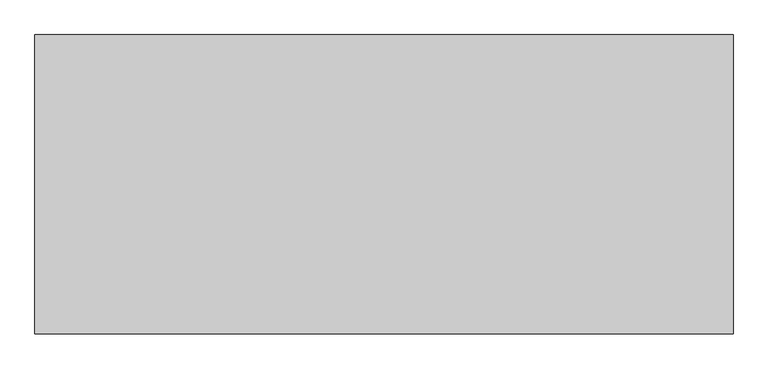
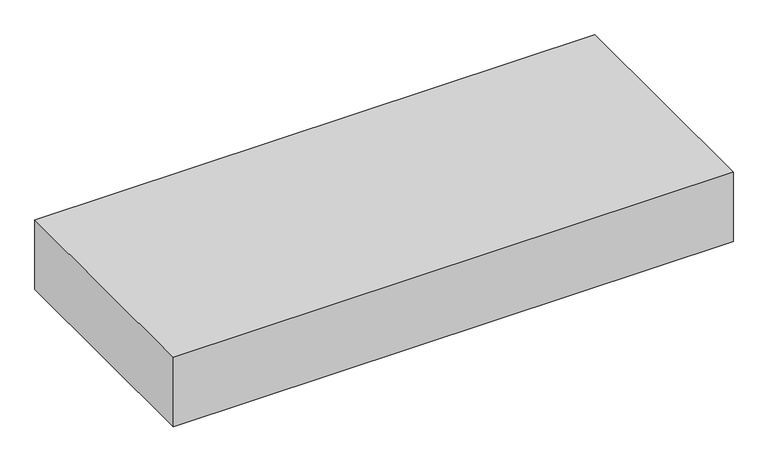
"""IFC4 building model written with IfcOpenShell, lengths in millimetres: proxy geometry, Space Planning Box_hec : Space Planning Box_hec."""

from ifc_helpers import new_model, si_unit, origin, origin_with_axes, place, context, project, spatial, polyline, outline, extrude, source, transform, mapped, element, save


def generic_models_3d03af35(model_context):
    return source(origin(), model_context, "Body", "SweptSolid", [
        extrude(outline(polyline([(21000.0, 9000.0), (21000.0, -9000.0), (-21000.0, -9000.0), (-21000.0, 9000.0), (21000.0, 9000.0)])), origin_with_axes(), (0.0, 0.0, 1.0), 5500.0),
    ])


if __name__ == "__main__":
    model = new_model("IFC4")
    model_context = context("Model", 3, world=origin())
    ifc_project = project(units=[si_unit("LENGTHUNIT", "METRE", prefix="MILLI")], contexts=[model_context])
    site = spatial("IfcSite", under=ifc_project)
    building = spatial("IfcBuilding", under=site)
    placement = place(None, origin())
    generic_models_shape = generic_models_3d03af35(model_context)
    element("IfcBuildingElementProxy", 1, Name="Space Planning Box_hec : Space Planning Box_hec", ObjectType="Space Planning Box_hec : Space Planning Box_hec", at=placement, inside=building, context=model_context, shape_type="MappedRepresentation", body=[
        mapped(generic_models_shape, transform((0.0, 0.0, 0.0), x_axis=(1.0, 0.0, 0.0), y_axis=(0.0, 1.0, 0.0), z_axis=(0.0, 0.0, 1.0))),
    ])
    save(model, "model.ifc")

# Revit data of these elements
# Type "Space Planning Box_hec : Space Planning Box_hec"
#   Type Comments = "..."
#   Room Name [instance default] = "?"
#   Interior Finish [instance default] = ""
#   Exterior Finish [instance default] = ""
#   Department [instance default] = ""
#   Assembly Code = "..."
#   ceiling height [instance default] = 0
#   Width [instance default] = 1524 mm
#   Program Area [instance default] = 0.00 m²
#   Length [instance default] = 1524 mm
#   Height [instance default] = 1524 mm
#   Area [instance default] = 2.32258 m²
#   Fill Color [instance default] = Cyan
#   Default Elevation = 0
# Element 1 (IfcBuildingElementProxy, "Space Planning Box_hec : Space Planning Box_hec")
#   Room Name = "Corridor"
#   Exterior Finish = "N/A..N/A,,EW2..N/A..N/A"
#   Department = "AR"
#   Width = 42000 mm
#   Length = 18000 mm
#   Height = 5500 mm
#   Area = 756.00 m²
#   Materials on its faces: "Cyan"
# Materials
#   "Cyan": class "Generic", colour RGB 0 255 255, transparency 0.2, Cost = 0
